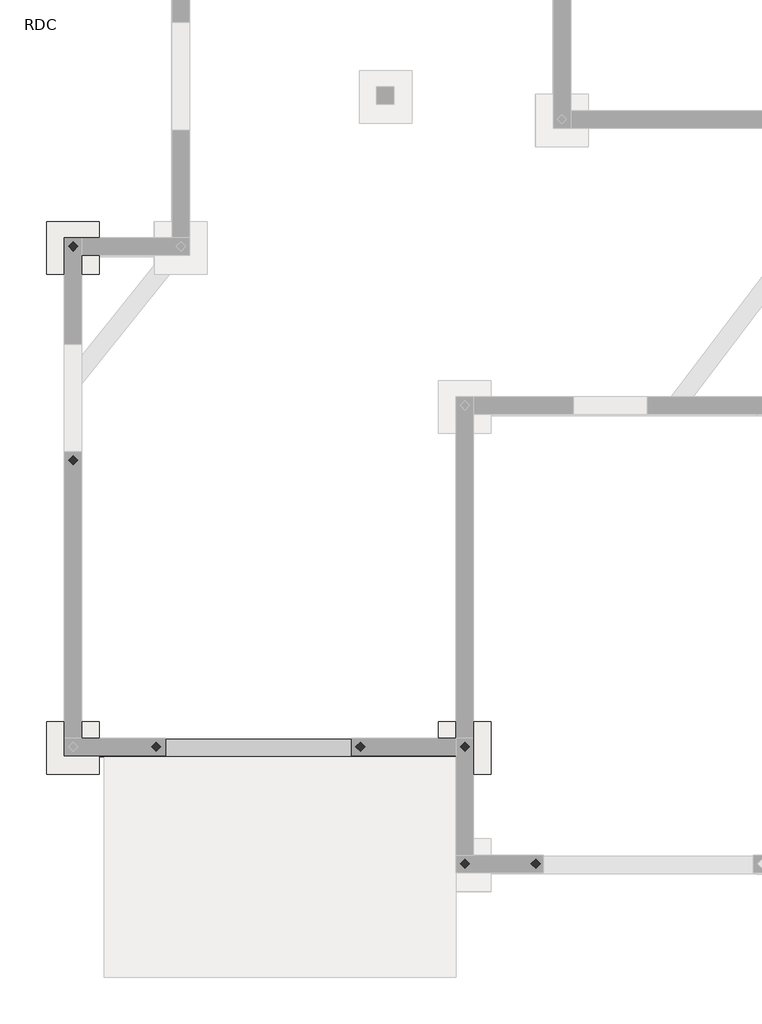
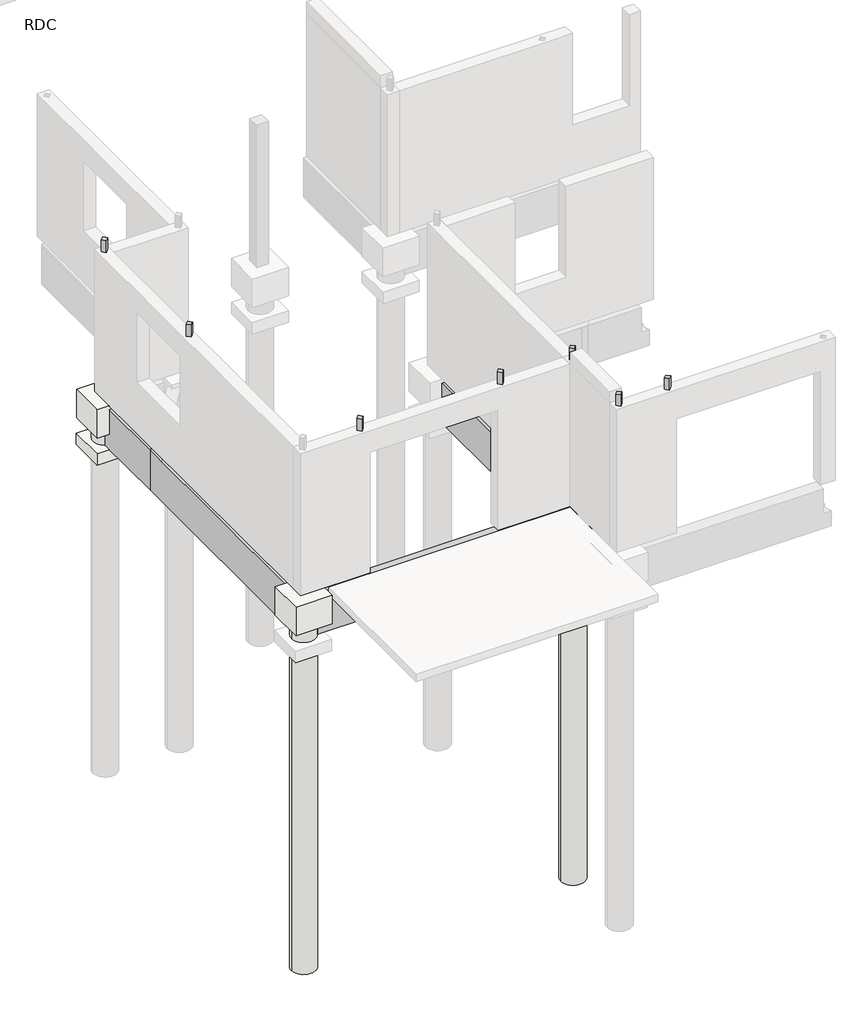
# One storey, part 2 of 5: 7 columns, 7 slabs, 5 beams.
"""IFC4 building model written with IfcOpenShell, lengths in millimetres."""

import ifcopenshell
import ifcopenshell.guid

model = None  # the IFC model being written
_history = None  # IfcOwnerHistory: only IFC2X3 demands one
_inside = {}  # id of a spatial element -> (the spatial element, [elements in it])
_under = {}  # id of a project, library or spatial element -> (it, [spatial elements below it])
_declared = {}  # id of a project -> (the project, [libraries it declares])
_typed = {}  # id of a type object -> (the type object, [elements of that type])
_made_of = {}  # id of a material, layer set ... -> (it, [elements and type objects made of it])


def new_model(schema):
    """Start an empty IFC model of exactly this schema.

    Asked for "IFC4X3", IfcOpenShell would pick the latest addendum, in which some entities
    have other attributes; the version numbers below select the first issue.
    IFC2X3 requires an IfcOwnerHistory on every rooted entity: one is made here for all.
    """
    global model, _history
    if schema == "IFC4X3":
        model = ifcopenshell.file(schema_version=(4, 3, 0, 0))
    else:
        model = ifcopenshell.file(schema=schema)
    _inside.clear()
    _under.clear()
    _declared.clear()
    _typed.clear()
    _made_of.clear()
    _history = None
    if model.schema == "IFC2X3":
        org = make("IfcOrganization", Name="unknown")
        user = make(
            "IfcPersonAndOrganization",
            ThePerson=make("IfcPerson", FamilyName="unknown"),
            TheOrganization=org,
        )
        app = make(
            "IfcApplication",
            ApplicationDeveloper=org,
            Version="unknown",
            ApplicationFullName="unknown",
            ApplicationIdentifier="unknown",
        )
        _history = make(
            "IfcOwnerHistory",
            OwningUser=user,
            OwningApplication=app,
            ChangeAction="ADDED",
            CreationDate=0,
        )
    return model


def make(cls, **values):
    """One entity of the class cls with the attributes given. An attribute that is None is left unset."""
    return model.create_entity(
        cls, **{name: value for name, value in values.items() if value is not None}
    )


def rooted(cls, **values):
    """An entity with a GlobalId (a new one), such as an element, a storey or a relation."""
    return make(cls, GlobalId=ifcopenshell.guid.new(), OwnerHistory=_history, **values)


def si_unit(unit_type, name, prefix=None):
    """IfcSIUnit, for example si_unit("LENGTHUNIT", "METRE", prefix="MILLI")."""
    return make("IfcSIUnit", UnitType=unit_type, Prefix=prefix, Name=name)


def assignment(units):
    """IfcUnitAssignment: the units of a project."""
    return None if units is None else make("IfcUnitAssignment", Units=units)


def point(xyz):
    """IfcCartesianPoint."""
    return None if xyz is None else make("IfcCartesianPoint", Coordinates=xyz)


def direction(xyz):
    """IfcDirection."""
    return None if xyz is None else make("IfcDirection", DirectionRatios=xyz)


def frame(location, z_axis=None, x_axis=None):
    """IfcAxis2Placement3D, a coordinate frame: its origin and axes. An axis left out is left unset."""
    return make(
        "IfcAxis2Placement3D",
        Location=point(location),
        Axis=direction(z_axis),
        RefDirection=direction(x_axis),
    )


def origin():
    """The frame at (0, 0, 0) with its axes left unset."""
    return frame((0.0, 0.0, 0.0))


def place(relative_to, where):
    """IfcLocalPlacement: puts the frame where relative to a parent placement (None: the world)."""
    return make(
        "IfcLocalPlacement", PlacementRelTo=relative_to, RelativePlacement=where
    )


def context(
    kind, dimensions, precision=None, world=None, true_north=None, identifier=None
):
    """IfcGeometricRepresentationContext, for example the 3D "Model" context."""
    return make(
        "IfcGeometricRepresentationContext",
        ContextIdentifier=identifier,
        ContextType=kind,
        CoordinateSpaceDimension=dimensions,
        Precision=precision,
        WorldCoordinateSystem=world,
        TrueNorth=true_north,
    )


def project(units=None, contexts=None):
    """IfcProject with its units and contexts."""
    return rooted(
        "IfcProject",
        Name="project",
        RepresentationContexts=contexts,
        UnitsInContext=assignment(units),
    )


def spatial(cls, under=None, at=None, **own):
    """A site, building, storey or space (cls), placed at a placement, below another one or the project."""
    s = rooted(cls, ObjectPlacement=at, **own)
    if under is not None:
        _under.setdefault(under.id(), (under, []))[1].append(s)
    return s


def polyline(points):
    """IfcPolyline through the points."""
    return make("IfcPolyline", Points=[point(p) for p in points])


def circle_curve(where, radius):
    """IfcCircle in the frame where."""
    return make("IfcCircle", Position=where, Radius=radius)


def outline(outer, holes=None, kind="AREA"):
    """IfcArbitraryClosedProfileDef: a profile drawn as a closed curve; with holes, ...WithVoids."""
    if holes is None:
        return make("IfcArbitraryClosedProfileDef", ProfileType=kind, OuterCurve=outer)
    return make(
        "IfcArbitraryProfileDefWithVoids",
        ProfileType=kind,
        OuterCurve=outer,
        InnerCurves=holes,
    )


def extrude(swept, where, along, depth):
    """IfcExtrudedAreaSolid: the profile swept, set in the frame where, extruded along a direction by depth."""
    return make(
        "IfcExtrudedAreaSolid",
        SweptArea=swept,
        Position=where,
        ExtrudedDirection=direction(along),
        Depth=depth,
    )


def faces_of(points, faces, orient=None, outer=None):
    """IfcFace entities. A face is a list of loops; a loop is a list of indices into points, from 0.

    orient and outer hold one flag for each loop. By default every Orientation is true, the
    first loop of a face is its IfcFaceOuterBound and the others are IfcFaceBound.
    """
    made = []
    for i, loops in enumerate(faces):
        bounds = []
        for j, loop in enumerate(loops):
            is_outer = j == 0 if outer is None else outer[i][j]
            bounds.append(
                make(
                    "IfcFaceOuterBound" if is_outer else "IfcFaceBound",
                    Bound=make("IfcPolyLoop", Polygon=[points[k] for k in loop]),
                    Orientation=True if orient is None else orient[i][j],
                )
            )
        made.append(make("IfcFace", Bounds=bounds))
    return made


def faceted_brep(points, faces, orient=None, outer=None, voids=None):
    """IfcFacetedBrep: a solid bounded by flat faces; with voids (closed shells), ...WithVoids."""
    shared = [point(p) for p in points]
    hull = make("IfcClosedShell", CfsFaces=faces_of(shared, faces, orient, outer))
    if voids is None:
        return make("IfcFacetedBrep", Outer=hull)
    return make(
        "IfcFacetedBrepWithVoids",
        Outer=hull,
        Voids=[
            make(cls, CfsFaces=faces_of(shared, fs, o, b)) for cls, fs, o, b in voids
        ],
    )


def shape(context_of_items, identifier, shape_type, items):
    """IfcShapeRepresentation: the items that make up one representation, for example the "Body"."""
    return make(
        "IfcShapeRepresentation",
        ContextOfItems=context_of_items,
        RepresentationIdentifier=identifier,
        RepresentationType=shape_type,
        Items=items,
    )


def made_of(thing, what):
    """Note that an element or type object is made of a material, layer set ...; save() writes the relation."""
    if what is not None:
        _made_of.setdefault(what.id(), (what, []))[1].append(thing)
    return thing


def element(
    cls,
    number,
    at=None,
    inside=None,
    cuts=None,
    type_object=None,
    material=None,
    context=None,
    identifier="Body",
    shape_type=None,
    held_by="IfcProductDefinitionShape",
    body=None,
    shapes=None,
    **own,
):
    """One element of the class cls, such as IfcWall. Its Tag is "e" and its number.

    at: its placement. inside: the storey or other place that contains it. cuts: it is an
    opening in that element (IfcRelVoidsElement). A single representation is given by context,
    identifier, shape_type and body (its items); several are given by shapes. held_by: the class
    of the entity that holds the representations. save() writes the other relations.
    """
    e = rooted(cls, Tag="e%d" % number, ObjectPlacement=at, **own)
    if body is not None:
        shapes = [shape(context, identifier, shape_type, body)]
    if shapes is not None:
        e.Representation = make(held_by, Representations=shapes)
    if inside is not None:
        _inside.setdefault(inside.id(), (inside, []))[1].append(e)
    if cuts is not None:
        rooted(
            "IfcRelVoidsElement", RelatingBuildingElement=cuts, RelatedOpeningElement=e
        )
    if type_object is not None:
        _typed.setdefault(type_object.id(), (type_object, []))[1].append(e)
    return made_of(e, material)


def aggregate(whole, parts):
    """IfcRelAggregates: a whole, such as a stair, and the parts it consists of."""
    return rooted("IfcRelAggregates", RelatingObject=whole, RelatedObjects=parts)


def save(model, path):
    """Write the relations noted so far, then the file.

    IfcRelAggregates (storeys below a building ...), IfcRelContainedInSpatialStructure (elements
    in a storey), IfcRelDefinesByType, IfcRelAssociatesMaterial and IfcRelDeclares: one each for
    every whole, place, type object, material and project.
    """
    for whole, parts in _under.values():
        aggregate(whole, parts)
    for where, things in _inside.values():
        rooted(
            "IfcRelContainedInSpatialStructure",
            RelatedElements=things,
            RelatingStructure=where,
        )
    for kind, things in _typed.values():
        rooted("IfcRelDefinesByType", RelatedObjects=things, RelatingType=kind)
    for what, things in _made_of.values():
        rooted("IfcRelAssociatesMaterial", RelatedObjects=things, RelatingMaterial=what)
    for by, libraries in _declared.values():
        rooted("IfcRelDeclares", RelatingContext=by, RelatedDefinitions=libraries)
    model.write(path)


def plane_surface(at):
    """IfcPlane: the flat surface through the origin of the frame at, square to its z axis."""
    return make("IfcPlane", Position=at)


def cylinder_surface(at, radius):
    """IfcCylindricalSurface: all points at the distance radius from the z axis of the frame at."""
    return make("IfcCylindricalSurface", Position=at, Radius=radius)


def revolved_surface(curve, axis_point, axis_direction):
    """IfcSurfaceOfRevolution: the curve turned about the line through axis_point along axis_direction."""
    return make(
        "IfcSurfaceOfRevolution",
        SweptCurve=make("IfcArbitraryOpenProfileDef", ProfileType="CURVE", Curve=curve),
        AxisPosition=make("IfcAxis1Placement", Location=point(axis_point), Axis=direction(axis_direction)),
    )


def advanced_brep(points, edges, surfaces, faces):
    """IfcAdvancedBrep: a solid bounded by faces that lie on surfaces and meet in shared edges.

    An edge is (start, end): straight between two places in points (the first is 0);
    or (start, end, curve); or (start, end, curve, False) where it runs against its curve.
    A face is (place in surfaces, loops), or (place, loops, False) where it looks against
    its surface's normal. A loop lists edges by number (the first is 1), with a minus sign
    where the edge is run from its end to its start. The first loop is the outer one.
    """
    corners = [point(p) for p in points]
    vertices = [make("IfcVertexPoint", VertexGeometry=c) for c in corners]
    made = []
    for start, end, *more in edges:
        made.append(
            make(
                "IfcEdgeCurve",
                EdgeStart=vertices[start],
                EdgeEnd=vertices[end],
                EdgeGeometry=more[0] if more else make("IfcPolyline", Points=[corners[start], corners[end]]),
                SameSense=more[1] if len(more) > 1 else True,
            )
        )
    hull = []
    for where, loops, *sense in faces:
        bounds = []
        for j, loop in enumerate(loops):
            ring = [make("IfcOrientedEdge", EdgeElement=made[abs(k) - 1], Orientation=k > 0) for k in loop]
            bounds.append(
                make(
                    "IfcFaceOuterBound" if j == 0 else "IfcFaceBound",
                    Bound=make("IfcEdgeLoop", EdgeList=ring),
                    Orientation=True,
                )
            )
        hull.append(make("IfcAdvancedFace", Bounds=bounds, FaceSurface=surfaces[where], SameSense=sense[0] if sense else True))
    return make("IfcAdvancedBrep", Outer=make("IfcClosedShell", CfsFaces=hull))


model = new_model("IFC4")

# Units and contexts
model_context = context("Model", 3, world=origin())
ifc_project = project(units=[si_unit("LENGTHUNIT", "METRE", prefix="MILLI")], contexts=[model_context])

# Site, building, storey
site = spatial("IfcSite", under=ifc_project)
building = spatial("IfcBuilding", under=site)
storey = spatial("IfcBuildingStorey", under=building, Name="RDC", Elevation=0.0)

# Beams
placement = place(None, origin())
element("IfcBeam", 1, ObjectType="Longrine BA : 20x70ht", at=placement, inside=storey, context=model_context, shape_type="AdvancedBrep", body=[
    advanced_brep(
    [(-6046.4904447, -2179.5386223, -767.0), (-6046.4904447, -2179.5386223, -67.0), (-6046.4904447, -6364.5149728, -67.0), (-6046.4904447, -6364.5149728, -500.0), (-6046.4904447, -6491.309892, -500.0), (-6046.4904447, -6491.309892, -767.0), (-6246.4904447, -6491.309892, -767.0), (-6246.4904447, -2429.4243416, -767.0), (-6246.4904447, -2429.4243416, -67.0), (-6246.4904447, -6491.309892, -500.0), (-6246.4904447, -6364.5149728, -500.0), (-6246.4904447, -6364.5149728, -67.0)],
    [
        (0, 1),
        (1, 2),
        (2, 3),
        (3, 4),
        (4, 5),
        (5, 0),
        (5, 6, circle_curve(frame((-6146.4904447, -6664.5149728, -767.0), z_axis=(0.0, 0.0, 1.0), x_axis=(1.0, 0.0, 0.0)), 200.0)),
        (6, 7),
        (7, 0),
        (8, 7),
        (6, 9),
        (9, 10),
        (10, 11),
        (11, 8),
        (1, 8),
        (11, 2),
        (4, 9, circle_curve(frame((-6146.4904447, -6664.5149728, -500.0), z_axis=(0.0, 0.0, 1.0), x_axis=(1.0, 0.0, 0.0)), 200.0)),
        (3, 10),
    ],
    [
        plane_surface(frame((-6046.4904447, -2539.7018932, -67.0), z_axis=(1.0, 0.0, 0.0), x_axis=(0.0, -1.0, 0.0))),
        plane_surface(frame((-6046.4904447, -2539.7018932, -767.0), z_axis=(0.0, 0.0, -1.0), x_axis=(0.0, -1.0, 0.0))),
        plane_surface(frame((-6246.4904447, -2539.7018932, -767.0), z_axis=(-1.0, 0.0, 0.0), x_axis=(0.0, -1.0, 0.0))),
        plane_surface(frame((-6246.4904447, -2539.7018932, -67.0), z_axis=(0.0, 0.0, 1.0), x_axis=(0.0, -1.0, 0.0))),
        revolved_surface(polyline([(-5946.4904447, -6664.5149728, -500.0), (-5946.4904447, -6664.5149728, -767.0)]), (-6146.4904447, -6664.5149728, -6600.0), (0.0, 0.0, 1.0)),
        plane_surface(frame((-6035.9796689, -2166.4061585, -767.0), z_axis=(-0.7807294524755704, 0.6248692039436703, 0.0), x_axis=(-0.6248692039436703, -0.7807294524755704, 0.0))),
        plane_surface(frame((-6446.4904447, -6364.5149728, -500.0), z_axis=(0.0, 0.0, 1.0), x_axis=(1.0, 0.0, 0.0))),
        plane_surface(frame((-5846.4904447, -6364.5149728, 0.0), z_axis=(0.0, -1.0, 0.0), x_axis=(0.0, 0.0, -1.0))),
    ],
    [
        (0, [[1, 2, 3, 4, 5, 6]]),
        (1, [[7, 8, 9, -6]]),
        (2, [[10, -8, 11, 12, 13, 14]]),
        (3, [[15, -14, 16, -2]]),
        (4, [[-7, -5, 17, -11]]),
        (5, [[-1, -9, -10, -15]]),
        (6, [[18, -12, -17, -4]]),
        (7, [[-18, -3, -16, -13]]),
    ],
),
])
element("IfcBeam", 2, ObjectType="Longrine BA : 20x70ht", at=placement, inside=storey, context=model_context, shape_type="AdvancedBrep", body=[
    advanced_brep(
    [(-1766.4904447, -6491.309892, -767.0), (-1766.4904447, -6491.309892, -500.0), (-1766.4904447, -6364.5149728, -500.0), (-1766.4904447, -6364.5149728, -67.0), (-1766.4904447, -3064.5149728, -67.0), (-1766.4904447, -3064.5149728, -500.0), (-1766.4904447, -2937.7200535, -500.0), (-1766.4904447, -2937.7200535, -767.0), (-1566.4904447, -6491.309892, -767.0), (-1566.4904447, -2937.7200535, -767.0), (-1566.4904447, -6491.309892, -500.0), (-1566.4904447, -2937.7200535, -500.0), (-1566.4904447, -3064.5149728, -500.0), (-1566.4904447, -3064.5149728, -67.0), (-1566.4904447, -6364.5149728, -67.0), (-1566.4904447, -6364.5149728, -500.0)],
    [
        (0, 1),
        (1, 2),
        (2, 3),
        (3, 4),
        (4, 5),
        (5, 6),
        (6, 7),
        (7, 0),
        (8, 0, circle_curve(frame((-1666.4904447, -6664.5149728, -767.0), z_axis=(0.0, 0.0, 1.0), x_axis=(1.0, 0.0, 0.0)), 200.0)),
        (7, 9, circle_curve(frame((-1666.4904447, -2764.5149728, -767.0), z_axis=(0.0, 0.0, 1.0), x_axis=(1.0, 0.0, 0.0)), 200.0)),
        (9, 8),
        (10, 8),
        (9, 11),
        (11, 12),
        (12, 13),
        (13, 14),
        (14, 15),
        (15, 10),
        (3, 14),
        (13, 4),
        (10, 1, circle_curve(frame((-1666.4904447, -6664.5149728, -500.0), z_axis=(0.0, 0.0, 1.0), x_axis=(1.0, 0.0, 0.0)), 200.0)),
        (6, 11, circle_curve(frame((-1666.4904447, -2764.5149728, -500.0), z_axis=(0.0, 0.0, 1.0), x_axis=(1.0, 0.0, 0.0)), 200.0)),
        (15, 2),
        (5, 12),
    ],
    [
        plane_surface(frame((-1766.4904447, -6649.277519, -417.0), z_axis=(-1.0, 0.0, 0.0), x_axis=(0.0, 0.0, -1.0))),
        plane_surface(frame((-1666.4904447, -6649.277519, -767.0), z_axis=(0.0, 0.0, -1.0), x_axis=(1.0, 0.0, 0.0))),
        plane_surface(frame((-1566.4904447, -6649.277519, -417.0), z_axis=(1.0, 0.0, 0.0), x_axis=(0.0, 0.0, 1.0))),
        plane_surface(frame((-1666.4904447, -6649.277519, -67.0), z_axis=(0.0, 0.0, 1.0), x_axis=(-1.0, 0.0, 0.0))),
        revolved_surface(polyline([(-1466.4904447, -6664.5149728, -500.0), (-1466.4904447, -6664.5149728, -767.0)]), (-1666.4904447, -6664.5149728, -6600.0), (0.0, 0.0, 1.0)),
        revolved_surface(polyline([(-1466.4904447, -2764.5149728, -500.0), (-1466.4904447, -2764.5149728, -767.0)]), (-1666.4904447, -2764.5149728, -6600.0), (0.0, 0.0, 1.0)),
        plane_surface(frame((-1966.4904447, -6364.5149728, -500.0), z_axis=(0.0, 0.0, 1.0), x_axis=(1.0, 0.0, 0.0))),
        plane_surface(frame((-1366.4904447, -6364.5149728, 0.0), z_axis=(0.0, -1.0, 0.0), x_axis=(0.0, 0.0, -1.0))),
        plane_surface(frame((-1966.4904447, -2464.5149728, -500.0), z_axis=(0.0, 0.0, 1.0), x_axis=(1.0, 0.0, 0.0))),
        plane_surface(frame((-1966.4904447, -3064.5149728, 0.0), z_axis=(0.0, 1.0, 0.0), x_axis=(0.0, 0.0, -1.0))),
    ],
    [
        (0, [[1, 2, 3, 4, 5, 6, 7, 8]]),
        (1, [[9, -8, 10, 11]]),
        (2, [[12, -11, 13, 14, 15, 16, 17, 18]]),
        (3, [[19, -16, 20, -4]]),
        (4, [[-1, -9, -12, 21]]),
        (5, [[-10, -7, 22, -13]]),
        (6, [[23, -2, -21, -18]]),
        (7, [[-23, -17, -19, -3]]),
        (8, [[24, -14, -22, -6]]),
        (9, [[-24, -5, -20, -15]]),
    ],
),
])
element("IfcBeam", 3, ObjectType="Longrine BA : 20x70ht", at=placement, inside=storey, context=model_context, shape_type="AdvancedBrep", body=[
    advanced_brep(
    [(-1766.4904447, -7828.7724377, -500.0), (-1766.4904447, -7701.9775185, -500.0), (-1766.4904447, -7701.9775185, -67.0), (-1766.4904447, -6964.5149728, -67.0), (-1766.4904447, -6964.5149728, -500.0), (-1766.4904447, -6837.7200535, -500.0), (-1766.4904447, -6837.7200535, -767.0), (-1766.4904447, -7828.7724377, -767.0), (-1566.4904447, -6837.7200535, -767.0), (-1566.4904447, -7828.7724377, -767.0), (-1566.4904447, -7828.7724377, -500.0), (-1566.4904447, -6837.7200535, -500.0), (-1566.4904447, -6964.5149728, -500.0), (-1566.4904447, -6964.5149728, -67.0), (-1566.4904447, -7701.9775185, -67.0), (-1566.4904447, -7701.9775185, -500.0)],
    [
        (0, 1),
        (1, 2),
        (2, 3),
        (3, 4),
        (4, 5),
        (5, 6),
        (6, 7),
        (7, 0),
        (6, 8, circle_curve(frame((-1666.4904447, -6664.5149728, -767.0), z_axis=(0.0, 0.0, 1.0), x_axis=(1.0, 0.0, 0.0)), 200.0)),
        (8, 9),
        (9, 7, circle_curve(frame((-1666.4904447, -8001.9775185, -767.0), z_axis=(0.0, 0.0, 1.0), x_axis=(1.0, 0.0, 0.0)), 200.0)),
        (10, 9),
        (8, 11),
        (11, 12),
        (12, 13),
        (13, 14),
        (14, 15),
        (15, 10),
        (2, 14),
        (13, 3),
        (5, 11, circle_curve(frame((-1666.4904447, -6664.5149728, -500.0), z_axis=(0.0, 0.0, 1.0), x_axis=(1.0, 0.0, 0.0)), 200.0)),
        (10, 0, circle_curve(frame((-1666.4904447, -8001.9775185, -500.0), z_axis=(0.0, 0.0, 1.0), x_axis=(1.0, 0.0, 0.0)), 200.0)),
        (15, 1),
        (4, 12),
    ],
    [
        plane_surface(frame((-1766.4904447, -7989.2775179, -417.0), z_axis=(-1.0, 0.0, 0.0), x_axis=(0.0, 0.0, -1.0))),
        plane_surface(frame((-1666.4904447, -7989.2775179, -767.0), z_axis=(0.0, 0.0, -1.0), x_axis=(1.0, 0.0, 0.0))),
        plane_surface(frame((-1566.4904447, -7989.2775179, -417.0), z_axis=(1.0, 0.0, 0.0), x_axis=(0.0, 0.0, 1.0))),
        plane_surface(frame((-1666.4904447, -7989.2775179, -67.0), z_axis=(0.0, 0.0, 1.0), x_axis=(-1.0, 0.0, 0.0))),
        revolved_surface(polyline([(-1466.4904447, -6664.5149728, -500.0), (-1466.4904447, -6664.5149728, -767.0)]), (-1666.4904447, -6664.5149728, -6600.0), (0.0, 0.0, 1.0)),
        revolved_surface(polyline([(-1466.4904447, -8001.9775185, -500.0), (-1466.4904447, -8001.9775185, -767.0)]), (-1666.4904447, -8001.9775185, -6600.0), (0.0, 0.0, 1.0)),
        plane_surface(frame((-1966.4904447, -7701.9775185, -500.0), z_axis=(0.0, 0.0, 1.0), x_axis=(1.0, 0.0, 0.0))),
        plane_surface(frame((-1366.4904447, -7701.9775185, 0.0), z_axis=(0.0, -1.0, 0.0), x_axis=(0.0, 0.0, -1.0))),
        plane_surface(frame((-1966.4904447, -6364.5149728, -500.0), z_axis=(0.0, 0.0, 1.0), x_axis=(1.0, 0.0, 0.0))),
        plane_surface(frame((-1966.4904447, -6964.5149728, 0.0), z_axis=(0.0, 1.0, 0.0), x_axis=(0.0, 0.0, -1.0))),
    ],
    [
        (0, [[1, 2, 3, 4, 5, 6, 7, 8]]),
        (1, [[9, 10, 11, -7]]),
        (2, [[12, -10, 13, 14, 15, 16, 17, 18]]),
        (3, [[19, -16, 20, -3]]),
        (4, [[-9, -6, 21, -13]]),
        (5, [[-12, 22, -8, -11]]),
        (6, [[23, -1, -22, -18]]),
        (7, [[-23, -17, -19, -2]]),
        (8, [[24, -14, -21, -5]]),
        (9, [[-24, -4, -20, -15]]),
    ],
),
])
element("IfcBeam", 4, ObjectType="Longrine BA : 20x70ht", at=placement, inside=storey, context=model_context, shape_type="AdvancedBrep", body=[
    advanced_brep(
    [(-5974.7753589, -6561.9775197, -767.0), (-5974.7753589, -6561.9775197, -500.0), (-5846.4904447, -6561.9775197, -500.0), (-5846.4904447, -6561.9775197, -67.0), (-1966.4904447, -6561.9775197, -67.0), (-1966.4904447, -6561.9775197, -500.0), (-1838.2055306, -6561.9775197, -500.0), (-1838.2055306, -6561.9775197, -767.0), (-5971.844941, -6761.9775197, -767.0), (-5946.4904447, -6664.5149728, -767.0), (-1866.4904447, -6664.5149728, -767.0), (-1841.1359484, -6761.9775197, -767.0), (-5971.844941, -6761.9775197, -500.0), (-1841.1359484, -6761.9775197, -500.0), (-1966.4904447, -6761.9775197, -500.0), (-1966.4904447, -6761.9775197, -130.0), (-1966.4904447, -6761.9775197, -67.0), (-5789.9771448, -6761.9775197, -67.0), (-5846.4904447, -6761.9775197, -67.0), (-5846.4904447, -6761.9775197, -500.0), (-5946.4904447, -6664.5149728, -500.0), (-1866.4904447, -6664.5149728, -500.0)],
    [
        (0, 1),
        (1, 2),
        (2, 3),
        (3, 4),
        (4, 5),
        (5, 6),
        (6, 7),
        (7, 0),
        (8, 9, circle_curve(frame((-6146.4904447, -6664.5149728, -767.0), z_axis=(0.0, 0.0, 1.0), x_axis=(1.0, 0.0, 0.0)), 200.0)),
        (9, 0, circle_curve(frame((-6146.4904447, -6664.5149728, -767.0), z_axis=(0.0, 0.0, 1.0), x_axis=(1.0, 0.0, 0.0)), 200.0)),
        (7, 10, circle_curve(frame((-1666.4904447, -6664.5149728, -767.0), z_axis=(0.0, 0.0, 1.0), x_axis=(1.0, 0.0, 0.0)), 200.0)),
        (10, 11, circle_curve(frame((-1666.4904447, -6664.5149728, -767.0), z_axis=(0.0, 0.0, 1.0), x_axis=(1.0, 0.0, 0.0)), 200.0)),
        (11, 8),
        (12, 8),
        (11, 13),
        (13, 14),
        (14, 15),
        (15, 16),
        (16, 17),
        (17, 18),
        (18, 19),
        (19, 12),
        (3, 18),
        (16, 4),
        (12, 20, circle_curve(frame((-6146.4904447, -6664.5149728, -500.0), z_axis=(0.0, 0.0, 1.0), x_axis=(1.0, 0.0, 0.0)), 200.0)),
        (20, 9),
        (20, 1, circle_curve(frame((-6146.4904447, -6664.5149728, -500.0), z_axis=(0.0, 0.0, 1.0), x_axis=(1.0, 0.0, 0.0)), 200.0)),
        (10, 21),
        (21, 13, circle_curve(frame((-1666.4904447, -6664.5149728, -500.0), z_axis=(0.0, 0.0, 1.0), x_axis=(1.0, 0.0, 0.0)), 200.0)),
        (6, 21, circle_curve(frame((-1666.4904447, -6664.5149728, -500.0), z_axis=(0.0, 0.0, 1.0), x_axis=(1.0, 0.0, 0.0)), 200.0)),
        (19, 2),
        (5, 14),
    ],
    [
        plane_surface(frame((-6133.7904441, -6561.9775197, -417.0), z_axis=(0.0, 1.0, 0.0), x_axis=(0.0, 0.0, -1.0))),
        plane_surface(frame((-6133.7904441, -6661.9775197, -767.0), z_axis=(0.0, 0.0, -1.0), x_axis=(0.0, -1.0, 0.0))),
        plane_surface(frame((-6133.7904441, -6761.9775197, -417.0), z_axis=(0.0, -1.0, 0.0), x_axis=(0.0, 0.0, 1.0))),
        plane_surface(frame((-6133.7904441, -6661.9775197, -67.0), z_axis=(0.0, 0.0, 1.0), x_axis=(0.0, 1.0, 0.0))),
        revolved_surface(polyline([(-5946.4904447, -6664.5149728, -500.0), (-5946.4904447, -6664.5149728, -767.0)]), (-6146.4904447, -6664.5149728, -6600.0), (0.0, 0.0, 1.0)),
        revolved_surface(polyline([(-1466.4904447, -6664.5149728, -500.0), (-1466.4904447, -6664.5149728, -767.0)]), (-1666.4904447, -6664.5149728, -6600.0), (0.0, 0.0, 1.0)),
        plane_surface(frame((-6446.4904447, -6364.5149728, -500.0), z_axis=(0.0, 0.0, 1.0), x_axis=(1.0, 0.0, 0.0))),
        plane_surface(frame((-5846.4904447, -6964.5149728, 0.0), z_axis=(-1.0, 0.0, 0.0), x_axis=(0.0, 0.0, -1.0))),
        plane_surface(frame((-1966.4904447, -6364.5149728, -500.0), z_axis=(0.0, 0.0, 1.0), x_axis=(1.0, 0.0, 0.0))),
        plane_surface(frame((-1966.4904447, -6364.5149728, 0.0), z_axis=(1.0, 0.0, 0.0), x_axis=(0.0, 0.0, -1.0))),
    ],
    [
        (0, [[1, 2, 3, 4, 5, 6, 7, 8]]),
        (1, [[9, 10, -8, 11, 12, 13]]),
        (2, [[14, -13, 15, 16, 17, 18, 19, 20, 21, 22]]),
        (3, [[23, -20, -19, 24, -4]]),
        (4, [[-14, 25, 26, -9]]),
        (4, [[-1, -10, -26, 27]]),
        (5, [[-12, 28, 29, -15]]),
        (5, [[-11, -7, 30, -28]]),
        (6, [[31, -2, -27, -25, -22]]),
        (7, [[-31, -21, -23, -3]]),
        (8, [[32, -16, -29, -30, -6]]),
        (9, [[-32, -5, -24, -18, -17]]),
    ],
),
])
element("IfcBeam", 5, ObjectType="Longrine BA : 20x70ht", at=placement, inside=storey, context=model_context, shape_type="AdvancedBrep", body=[
    advanced_brep(
    [(-6046.4904447, -1117.578479, -767.0), (-6046.4904447, -1117.578479, -500.0), (-6046.4904447, -1244.3733983, -500.0), (-6046.4904447, -1244.3733983, -67.0), (-6046.4904447, -2179.5386223, -67.0), (-6046.4904447, -2179.5386223, -767.0), (-6246.4904447, -1117.578479, -767.0), (-6246.4904447, -2429.4243416, -767.0), (-6246.4904447, -1117.578479, -500.0), (-6246.4904447, -2429.4243416, -67.0), (-6246.4904447, -1244.3733983, -67.0), (-6246.4904447, -1244.3733983, -500.0)],
    [
        (0, 1),
        (1, 2),
        (2, 3),
        (3, 4),
        (4, 5),
        (5, 0),
        (6, 0, circle_curve(frame((-6146.4904447, -944.3733983, -767.0), z_axis=(0.0, 0.0, 1.0), x_axis=(1.0, 0.0, 0.0)), 200.0)),
        (5, 7),
        (7, 6),
        (8, 6),
        (7, 9),
        (9, 10),
        (10, 11),
        (11, 8),
        (3, 10),
        (9, 4),
        (8, 1, circle_curve(frame((-6146.4904447, -944.3733983, -500.0), z_axis=(0.0, 0.0, 1.0), x_axis=(1.0, 0.0, 0.0)), 200.0)),
        (11, 2),
    ],
    [
        plane_surface(frame((-6046.4904447, -957.0734248, -67.0), z_axis=(1.0, 0.0, 0.0), x_axis=(0.0, -1.0, 0.0))),
        plane_surface(frame((-6046.4904447, -957.0734248, -767.0), z_axis=(0.0, 0.0, -1.0), x_axis=(0.0, -1.0, 0.0))),
        plane_surface(frame((-6246.4904447, -957.0734248, -767.0), z_axis=(-1.0, 0.0, 0.0), x_axis=(0.0, -1.0, 0.0))),
        plane_surface(frame((-6246.4904447, -957.0734248, -67.0), z_axis=(0.0, 0.0, 1.0), x_axis=(0.0, -1.0, 0.0))),
        revolved_surface(polyline([(-5946.4904447, -944.3733983, -500.0), (-5946.4904447, -944.3733983, -767.0)]), (-6146.4904447, -944.3733983, -6600.0), (0.0, 0.0, 1.0)),
        plane_surface(frame((-6446.4904447, -644.3733983, -500.0), z_axis=(0.0, 0.0, 1.0), x_axis=(1.0, 0.0, 0.0))),
        plane_surface(frame((-6446.4904447, -1244.3733983, 0.0), z_axis=(0.0, 1.0, 0.0), x_axis=(0.0, 0.0, -1.0))),
        plane_surface(frame((-6035.9796689, -2166.4061585, -767.0), z_axis=(0.7807294524755704, -0.6248692039436703, 0.0), x_axis=(-0.6248692039436703, -0.7807294524755704, 0.0))),
    ],
    [
        (0, [[1, 2, 3, 4, 5, 6]]),
        (1, [[7, -6, 8, 9]]),
        (2, [[10, -9, 11, 12, 13, 14]]),
        (3, [[15, -12, 16, -4]]),
        (4, [[-1, -7, -10, 17]]),
        (5, [[18, -2, -17, -14]]),
        (6, [[-18, -13, -15, -3]]),
        (7, [[-5, -16, -11, -8]]),
    ],
),
])

# Columns
element("IfcColumn", 6, ObjectType="CV : CV", at=placement, inside=storey, context=model_context, shape_type="Brep", body=[
    faceted_brep([(-1665.4336406, -6595.6690755, 2710.0), (-1718.4666492, -6648.7020841, 2710.0), (-1665.4336406, -6701.7350927, 2710.0), (-1612.400632, -6648.7020841, 2710.0), (-1665.4336406, -6595.6690755, 0.0), (-1612.400632, -6648.7020841, 0.0), (-1665.4336406, -6701.7350927, 0.0), (-1718.4666492, -6648.7020841, 0.0), (-1665.4336406, -6595.6690755, 2500.0), (-1718.4666492, -6648.7020841, 2500.0), (-1665.4336406, -6701.7350927, 2500.0), (-1612.400632, -6648.7020841, 2500.0)], [[[0, 1, 2, 3]], [[4, 5, 6, 7]], [[1, 0, 8, 4, 7, 9]], [[2, 1, 9, 7, 6, 10]], [[3, 2, 10, 6, 5, 11]], [[0, 3, 11, 5, 4, 8]]]),
    faceted_brep([(-1612.400632, -6648.7020841, 2710.0), (-1665.4336406, -6595.6690755, 2710.0), (-1718.4666492, -6648.7020841, 2710.0), (-1665.4336406, -6701.7350927, 2710.0), (-1612.400632, -6648.7020841, 0.0), (-1665.4336406, -6701.7350927, 0.0), (-1718.4666492, -6648.7020841, 0.0), (-1665.4336406, -6595.6690755, 0.0), (-1612.400632, -6648.7020841, 2500.0), (-1665.4336406, -6595.6690755, 2500.0), (-1718.4666492, -6648.7020841, 2500.0), (-1665.4336406, -6701.7350927, 2500.0)], [[[0, 1, 2, 3]], [[4, 5, 6, 7]], [[1, 0, 8, 4, 7, 9]], [[2, 1, 9, 7, 6, 10]], [[3, 2, 10, 6, 5, 11]], [[0, 3, 11, 5, 4, 8]]]),
])
element("IfcColumn", 7, ObjectType="CV : CV", at=placement, inside=storey, context=model_context, shape_type="Brep", body=[
    faceted_brep([(-855.4336191, -7933.1316212, 2710.0), (-908.4666277, -7986.1646298, 2710.0), (-855.4336191, -8039.1976384, 2710.0), (-802.4006105, -7986.1646298, 2710.0), (-855.4336191, -7933.1316212, 0.0), (-802.4006105, -7986.1646298, 0.0), (-855.4336191, -8039.1976384, 0.0), (-908.4666277, -7986.1646298, 0.0), (-855.4336191, -7933.1316212, 2510.0), (-908.4666277, -7986.1646298, 2510.0), (-855.4336191, -8039.1976384, 2510.0), (-802.4006105, -7986.1646298, 2510.0)], [[[0, 1, 2, 3]], [[4, 5, 6, 7]], [[1, 0, 8, 4, 7, 9]], [[2, 1, 9, 7, 6, 10]], [[3, 2, 10, 6, 5, 11]], [[0, 3, 11, 5, 4, 8]]]),
    faceted_brep([(-802.4006105, -7986.1646298, 2710.0), (-855.4336191, -7933.1316212, 2710.0), (-908.4666277, -7986.1646298, 2710.0), (-855.4336191, -8039.1976384, 2710.0), (-802.4006105, -7986.1646298, 0.0), (-855.4336191, -8039.1976384, 0.0), (-908.4666277, -7986.1646298, 0.0), (-855.4336191, -7933.1316212, 0.0), (-802.4006105, -7986.1646298, 2510.0), (-855.4336191, -7933.1316212, 2510.0), (-908.4666277, -7986.1646298, 2510.0), (-855.4336191, -8039.1976384, 2510.0)], [[[0, 1, 2, 3]], [[4, 5, 6, 7]], [[1, 0, 8, 4, 7, 9]], [[2, 1, 9, 7, 6, 10]], [[3, 2, 10, 6, 5, 11]], [[0, 3, 11, 5, 4, 8]]]),
])
element("IfcColumn", 8, ObjectType="CV : CV", at=placement, inside=storey, context=model_context, shape_type="Brep", body=[
    faceted_brep([(-1665.4336406, -7933.1316212, 2710.0), (-1718.4666492, -7986.1646298, 2710.0), (-1665.4336406, -8039.1976384, 2710.0), (-1612.400632, -7986.1646298, 2710.0), (-1665.4336406, -7933.1316212, 0.0), (-1612.400632, -7986.1646298, 0.0), (-1665.4336406, -8039.1976384, 0.0), (-1718.4666492, -7986.1646298, 0.0), (-1665.4336406, -7933.1316212, 2510.0), (-1718.4666492, -7986.1646298, 2510.0), (-1665.4336406, -8039.1976384, 2510.0), (-1612.400632, -7986.1646298, 2510.0)], [[[0, 1, 2, 3]], [[4, 5, 6, 7]], [[1, 0, 8, 4, 7, 9]], [[2, 1, 9, 7, 6, 10]], [[3, 2, 10, 6, 5, 11]], [[0, 3, 11, 5, 4, 8]]]),
    faceted_brep([(-1612.400632, -7986.1646298, 2710.0), (-1665.4336406, -7933.1316212, 2710.0), (-1718.4666492, -7986.1646298, 2710.0), (-1665.4336406, -8039.1976384, 2710.0), (-1612.400632, -7986.1646298, 0.0), (-1665.4336406, -8039.1976384, 0.0), (-1718.4666492, -7986.1646298, 0.0), (-1665.4336406, -7933.1316212, 0.0), (-1612.400632, -7986.1646298, 2510.0), (-1665.4336406, -7933.1316212, 2510.0), (-1718.4666492, -7986.1646298, 2510.0), (-1665.4336406, -8039.1976384, 2510.0)], [[[0, 1, 2, 3]], [[4, 5, 6, 7]], [[1, 0, 8, 4, 7, 9]], [[2, 1, 9, 7, 6, 10]], [[3, 2, 10, 6, 5, 11]], [[0, 3, 11, 5, 4, 8]]]),
])
element("IfcColumn", 9, ObjectType="CV : CV", at=placement, inside=storey, context=model_context, shape_type="Brep", body=[
    faceted_brep([(-2861.4904447, -6595.6690755, 2710.0), (-2914.5234533, -6648.7020841, 2710.0), (-2861.4904447, -6701.7350927, 2710.0), (-2808.4574361, -6648.7020841, 2710.0), (-2861.4904447, -6595.6690755, 0.0), (-2808.4574361, -6648.7020841, 0.0), (-2861.4904447, -6701.7350927, 0.0), (-2914.5234533, -6648.7020841, 0.0), (-2861.4904447, -6595.6690755, 2500.0), (-2914.5234533, -6648.7020841, 2500.0), (-2861.4904447, -6701.7350927, 2500.0), (-2808.4574361, -6648.7020841, 2500.0)], [[[0, 1, 2, 3]], [[4, 5, 6, 7]], [[1, 0, 8, 4, 7, 9]], [[2, 1, 9, 7, 6, 10]], [[3, 2, 10, 6, 5, 11]], [[0, 3, 11, 5, 4, 8]]]),
    faceted_brep([(-2808.4574361, -6648.7020841, 2710.0), (-2861.4904447, -6595.6690755, 2710.0), (-2914.5234533, -6648.7020841, 2710.0), (-2861.4904447, -6701.7350927, 2710.0), (-2808.4574361, -6648.7020841, 0.0), (-2861.4904447, -6701.7350927, 0.0), (-2914.5234533, -6648.7020841, 0.0), (-2861.4904447, -6595.6690755, 0.0), (-2808.4574361, -6648.7020841, 2500.0), (-2861.4904447, -6595.6690755, 2500.0), (-2914.5234533, -6648.7020841, 2500.0), (-2861.4904447, -6701.7350927, 2500.0)], [[[0, 1, 2, 3]], [[4, 5, 6, 7]], [[1, 0, 8, 4, 7, 9]], [[2, 1, 9, 7, 6, 10]], [[3, 2, 10, 6, 5, 11]], [[0, 3, 11, 5, 4, 8]]]),
])
element("IfcColumn", 10, ObjectType="CV : CV", at=placement, inside=storey, context=model_context, shape_type="Brep", body=[
    faceted_brep([(-5197.6214092, -6595.6690755, 2710.0), (-5250.6544178, -6648.7020841, 2710.0), (-5197.6214092, -6701.7350927, 2710.0), (-5144.5884006, -6648.7020841, 2710.0), (-5197.6214092, -6595.6690755, 0.0), (-5144.5884006, -6648.7020841, 0.0), (-5197.6214092, -6701.7350927, 0.0), (-5250.6544178, -6648.7020841, 0.0), (-5197.6214092, -6595.6690755, 2500.0), (-5250.6544178, -6648.7020841, 2500.0), (-5197.6214092, -6701.7350927, 2500.0), (-5144.5884006, -6648.7020841, 2500.0)], [[[0, 1, 2, 3]], [[4, 5, 6, 7]], [[1, 0, 8, 4, 7, 9]], [[2, 1, 9, 7, 6, 10]], [[3, 2, 10, 6, 5, 11]], [[0, 3, 11, 5, 4, 8]]]),
    faceted_brep([(-5144.5884006, -6648.7020841, 2710.0), (-5197.6214092, -6595.6690755, 2710.0), (-5250.6544178, -6648.7020841, 2710.0), (-5197.6214092, -6701.7350927, 2710.0), (-5144.5884006, -6648.7020841, 0.0), (-5197.6214092, -6701.7350927, 0.0), (-5250.6544178, -6648.7020841, 0.0), (-5197.6214092, -6595.6690755, 0.0), (-5144.5884006, -6648.7020841, 2500.0), (-5197.6214092, -6595.6690755, 2500.0), (-5250.6544178, -6648.7020841, 2500.0), (-5197.6214092, -6701.7350927, 2500.0)], [[[0, 1, 2, 3]], [[4, 5, 6, 7]], [[1, 0, 8, 4, 7, 9]], [[2, 1, 9, 7, 6, 10]], [[3, 2, 10, 6, 5, 11]], [[0, 3, 11, 5, 4, 8]]]),
])
element("IfcColumn", 11, ObjectType="CV : CV", at=placement, inside=storey, context=model_context, shape_type="Brep", body=[
    faceted_brep([(-6146.4904447, -3320.5275198, 2710.0), (-6199.5234533, -3373.5605284, 2710.0), (-6146.4904447, -3426.593537, 2710.0), (-6093.4574361, -3373.5605284, 2710.0), (-6146.4904447, -3320.5275198, 0.0), (-6093.4574361, -3373.5605284, 0.0), (-6146.4904447, -3426.593537, 0.0), (-6199.5234533, -3373.5605284, 0.0), (-6146.4904447, -3320.5275198, 2500.0), (-6199.5234533, -3373.5605284, 2500.0), (-6146.4904447, -3426.593537, 2500.0), (-6093.4574361, -3373.5605284, 2500.0)], [[[0, 1, 2, 3]], [[4, 5, 6, 7]], [[1, 0, 8, 4, 7, 9]], [[2, 1, 9, 7, 6, 10]], [[3, 2, 10, 6, 5, 11]], [[0, 3, 11, 5, 4, 8]]]),
    faceted_brep([(-6093.4574361, -3373.5605284, 2710.0), (-6146.4904447, -3320.5275198, 2710.0), (-6199.5234533, -3373.5605284, 2710.0), (-6146.4904447, -3426.593537, 2710.0), (-6093.4574361, -3373.5605284, 0.0), (-6146.4904447, -3426.593537, 0.0), (-6199.5234533, -3373.5605284, 0.0), (-6146.4904447, -3320.5275198, 0.0), (-6093.4574361, -3373.5605284, 2500.0), (-6146.4904447, -3320.5275198, 2500.0), (-6199.5234533, -3373.5605284, 2500.0), (-6146.4904447, -3426.593537, 2500.0)], [[[0, 1, 2, 3]], [[4, 5, 6, 7]], [[1, 0, 8, 4, 7, 9]], [[2, 1, 9, 7, 6, 10]], [[3, 2, 10, 6, 5, 11]], [[0, 3, 11, 5, 4, 8]]]),
])
element("IfcColumn", 12, ObjectType="CV : CV", at=placement, inside=storey, context=model_context, shape_type="Brep", body=[
    faceted_brep([(-6146.4904447, -875.527527, 2710.0), (-6199.5234533, -928.5605356, 2710.0), (-6146.4904447, -981.5935442, 2710.0), (-6093.4574361, -928.5605356, 2710.0), (-6146.4904447, -875.527527, 0.0), (-6093.4574361, -928.5605356, 0.0), (-6146.4904447, -981.5935442, 0.0), (-6199.5234533, -928.5605356, 0.0), (-6146.4904447, -875.527527, 2500.0), (-6199.5234533, -928.5605356, 2500.0), (-6146.4904447, -981.5935442, 2500.0), (-6093.4574361, -928.5605356, 2500.0)], [[[0, 1, 2, 3]], [[4, 5, 6, 7]], [[1, 0, 8, 4, 7, 9]], [[2, 1, 9, 7, 6, 10]], [[3, 2, 10, 6, 5, 11]], [[0, 3, 11, 5, 4, 8]]]),
    faceted_brep([(-6093.4574361, -928.5605356, 2710.0), (-6146.4904447, -875.527527, 2710.0), (-6199.5234533, -928.5605356, 2710.0), (-6146.4904447, -981.5935442, 2710.0), (-6093.4574361, -928.5605356, 0.0), (-6146.4904447, -981.5935442, 0.0), (-6199.5234533, -928.5605356, 0.0), (-6146.4904447, -875.527527, 0.0), (-6093.4574361, -928.5605356, 2500.0), (-6146.4904447, -875.527527, 2500.0), (-6199.5234533, -928.5605356, 2500.0), (-6146.4904447, -981.5935442, 2500.0)], [[[0, 1, 2, 3]], [[4, 5, 6, 7]], [[1, 0, 8, 4, 7, 9]], [[2, 1, 9, 7, 6, 10]], [[3, 2, 10, 6, 5, 11]], [[0, 3, 11, 5, 4, 8]]]),
])

# Slabs
element("IfcSlab", 13, ObjectType="Pieu-Conduite en acier : Diamètre de 400 mm", at=placement, inside=storey, context=model_context, shape_type="AdvancedBrep", body=[
    advanced_brep(
    [(-6346.4904447, -6664.5149728, -6600.0), (-5946.4904447, -6664.5149728, -6600.0), (-6346.4904447, -6664.5149728, -970.0), (-5946.4904447, -6664.5149728, -970.0)],
    [
        (0, 1, circle_curve(frame((-6146.4904447, -6664.5149728, -6600.0), z_axis=(0.0, 0.0, -1.0), x_axis=(1.0, 0.0, 0.0)), 200.0)),
        (1, 0, circle_curve(frame((-6146.4904447, -6664.5149728, -6600.0), z_axis=(0.0, 0.0, -1.0), x_axis=(1.0, 0.0, 0.0)), 200.0)),
        (2, 3, circle_curve(frame((-6146.4904447, -6664.5149728, -970.0), z_axis=(0.0, 0.0, 1.0), x_axis=(1.0, 0.0, 0.0)), 200.0)),
        (3, 2, circle_curve(frame((-6146.4904447, -6664.5149728, -970.0), z_axis=(0.0, 0.0, 1.0), x_axis=(1.0, 0.0, 0.0)), 200.0)),
        (1, 3),
        (2, 0),
    ],
    [
        plane_surface(frame((-5946.4904447, -6664.5149728, -6600.0), z_axis=(0.0, 0.0, -1.0), x_axis=(0.0, -1.0, 0.0))),
        plane_surface(frame((-6451.0339778, -6364.5149728, -970.0), z_axis=(0.0, 0.0, 1.0), x_axis=(1.0, 0.0, 0.0))),
        cylinder_surface(frame((-6146.4904447, -6664.5149728, -6600.0), z_axis=(0.0, 0.0, 1.0), x_axis=(1.0, 0.0, 0.0)), 200.0),
    ],
    [
        (0, [[1, 2]]),
        (1, [[3, 4]]),
        (2, [[-2, 5, -3, 6]]),
        (2, [[-1, -6, -4, -5]]),
    ],
),
    advanced_brep(
    [(-6346.4904447, -6664.5149728, -770.0), (-5946.4904447, -6664.5149728, -770.0), (-5946.4904447, -6664.5149728, -500.0), (-5971.844941, -6761.9775197, -500.0), (-6346.4904447, -6664.5149728, -500.0), (-6246.4904447, -6491.309892, -500.0), (-6046.4904447, -6491.309892, -500.0), (-5974.7836363, -6561.9636591, -500.0)],
    [
        (0, 1, circle_curve(frame((-6146.4904447, -6664.5149728, -770.0), z_axis=(0.0, 0.0, 1.0), x_axis=(1.0, 0.0, 0.0)), 200.0)),
        (1, 2),
        (2, 3, circle_curve(frame((-6146.4904447, -6664.5149728, -500.0), z_axis=(0.0, 0.0, -1.0), x_axis=(1.0, 0.0, 0.0)), 200.0)),
        (3, 4, circle_curve(frame((-6146.4904447, -6664.5149728, -500.0), z_axis=(0.0, 0.0, -1.0), x_axis=(1.0, 0.0, 0.0)), 200.0)),
        (4, 0),
        (1, 0, circle_curve(frame((-6146.4904447, -6664.5149728, -770.0), z_axis=(0.0, 0.0, 1.0), x_axis=(1.0, 0.0, 0.0)), 200.0)),
        (4, 5, circle_curve(frame((-6146.4904447, -6664.5149728, -500.0), z_axis=(0.0, 0.0, -1.0), x_axis=(1.0, 0.0, 0.0)), 200.0)),
        (5, 6, circle_curve(frame((-6146.4904447, -6664.5149728, -500.0), z_axis=(0.0, 0.0, -1.0), x_axis=(1.0, 0.0, 0.0)), 200.0)),
        (6, 7, circle_curve(frame((-6146.4904447, -6664.5149728, -500.0), z_axis=(0.0, 0.0, -1.0), x_axis=(1.0, 0.0, 0.0)), 200.0)),
        (7, 2, circle_curve(frame((-6146.4904447, -6664.5149728, -500.0), z_axis=(0.0, 0.0, -1.0), x_axis=(1.0, 0.0, 0.0)), 200.0)),
    ],
    [
        cylinder_surface(frame((-6146.4904447, -6664.5149728, -6600.0), z_axis=(0.0, 0.0, 1.0), x_axis=(1.0, 0.0, 0.0)), 200.0),
        plane_surface(frame((-6451.0339778, -6364.5149728, -770.0), z_axis=(0.0, 0.0, -1.0), x_axis=(-1.0, 0.0, 0.0))),
        plane_surface(frame((-6446.4904447, -6364.5149728, -500.0), z_axis=(0.0, 0.0, 1.0), x_axis=(1.0, 0.0, 0.0))),
    ],
    [
        (0, [[1, 2, 3, 4, 5]]),
        (0, [[6, -5, 7, 8, 9, 10, -2]]),
        (1, [[-1, -6]]),
        (2, [[-4, -3, -10, -9, -8, -7]]),
    ],
),
])
element("IfcSlab", 14, ObjectType="Pieu-Conduite en acier : Diamètre de 400 mm", at=placement, inside=storey, context=model_context, shape_type="AdvancedBrep", body=[
    advanced_brep(
    [(-1866.4904447, -6664.5149728, -6600.0), (-1466.4904447, -6664.5149728, -6600.0), (-1866.4904447, -6664.5149728, -970.0), (-1466.4904447, -6664.5149728, -970.0)],
    [
        (0, 1, circle_curve(frame((-1666.4904447, -6664.5149728, -6600.0), z_axis=(0.0, 0.0, -1.0), x_axis=(1.0, 0.0, 0.0)), 200.0)),
        (1, 0, circle_curve(frame((-1666.4904447, -6664.5149728, -6600.0), z_axis=(0.0, 0.0, -1.0), x_axis=(1.0, 0.0, 0.0)), 200.0)),
        (2, 3, circle_curve(frame((-1666.4904447, -6664.5149728, -970.0), z_axis=(0.0, 0.0, 1.0), x_axis=(1.0, 0.0, 0.0)), 200.0)),
        (3, 2, circle_curve(frame((-1666.4904447, -6664.5149728, -970.0), z_axis=(0.0, 0.0, 1.0), x_axis=(1.0, 0.0, 0.0)), 200.0)),
        (1, 3),
        (2, 0),
    ],
    [
        plane_surface(frame((-1466.4904447, -6664.5149728, -6600.0), z_axis=(0.0, 0.0, -1.0), x_axis=(0.0, -1.0, 0.0))),
        plane_surface(frame((-1969.9771566, -6364.5149728, -970.0), z_axis=(0.0, 0.0, 1.0), x_axis=(1.0, 0.0, 0.0))),
        cylinder_surface(frame((-1666.4904447, -6664.5149728, -6600.0), z_axis=(0.0, 0.0, 1.0), x_axis=(1.0, 0.0, 0.0)), 200.0),
    ],
    [
        (0, [[1, 2]]),
        (1, [[3, 4]]),
        (2, [[-2, 5, -3, 6]]),
        (2, [[-1, -6, -4, -5]]),
    ],
),
    advanced_brep(
    [(-1866.4904447, -6664.5149728, -770.0), (-1466.4904447, -6664.5149728, -770.0), (-1466.4904447, -6664.5149728, -500.0), (-1566.4904447, -6837.7200535, -500.0), (-1766.4904447, -6837.7200535, -500.0), (-1841.127419, -6761.9928022, -500.0), (-1866.4904447, -6664.5149728, -500.0), (-1838.1972532, -6561.9636591, -500.0), (-1766.4904447, -6491.309892, -500.0), (-1566.4904447, -6491.309892, -500.0)],
    [
        (0, 1, circle_curve(frame((-1666.4904447, -6664.5149728, -770.0), z_axis=(0.0, 0.0, 1.0), x_axis=(1.0, 0.0, 0.0)), 200.0)),
        (1, 2),
        (2, 3, circle_curve(frame((-1666.4904447, -6664.5149728, -500.0), z_axis=(0.0, 0.0, -1.0), x_axis=(1.0, 0.0, 0.0)), 200.0)),
        (3, 4, circle_curve(frame((-1666.4904447, -6664.5149728, -500.0), z_axis=(0.0, 0.0, -1.0), x_axis=(1.0, 0.0, 0.0)), 200.0)),
        (4, 5, circle_curve(frame((-1666.4904447, -6664.5149728, -500.0), z_axis=(0.0, 0.0, -1.0), x_axis=(1.0, 0.0, 0.0)), 200.0)),
        (5, 6, circle_curve(frame((-1666.4904447, -6664.5149728, -500.0), z_axis=(0.0, 0.0, -1.0), x_axis=(1.0, 0.0, 0.0)), 200.0)),
        (6, 0),
        (1, 0, circle_curve(frame((-1666.4904447, -6664.5149728, -770.0), z_axis=(0.0, 0.0, 1.0), x_axis=(1.0, 0.0, 0.0)), 200.0)),
        (6, 7, circle_curve(frame((-1666.4904447, -6664.5149728, -500.0), z_axis=(0.0, 0.0, -1.0), x_axis=(1.0, 0.0, 0.0)), 200.0)),
        (7, 8, circle_curve(frame((-1666.4904447, -6664.5149728, -500.0), z_axis=(0.0, 0.0, -1.0), x_axis=(1.0, 0.0, 0.0)), 200.0)),
        (8, 9, circle_curve(frame((-1666.4904447, -6664.5149728, -500.0), z_axis=(0.0, 0.0, -1.0), x_axis=(1.0, 0.0, 0.0)), 200.0)),
        (9, 2, circle_curve(frame((-1666.4904447, -6664.5149728, -500.0), z_axis=(0.0, 0.0, -1.0), x_axis=(1.0, 0.0, 0.0)), 200.0)),
    ],
    [
        cylinder_surface(frame((-1666.4904447, -6664.5149728, -6600.0), z_axis=(0.0, 0.0, 1.0), x_axis=(1.0, 0.0, 0.0)), 200.0),
        plane_surface(frame((-1969.9771566, -6364.5149728, -770.0), z_axis=(0.0, 0.0, -1.0), x_axis=(-1.0, 0.0, 0.0))),
        plane_surface(frame((-1966.4904447, -6364.5149728, -500.0), z_axis=(0.0, 0.0, 1.0), x_axis=(1.0, 0.0, 0.0))),
    ],
    [
        (0, [[1, 2, 3, 4, 5, 6, 7]]),
        (0, [[8, -7, 9, 10, 11, 12, -2]]),
        (1, [[-1, -8]]),
        (2, [[-6, -5, -4, -3, -12, -11, -10, -9]]),
    ],
),
])
element("IfcSlab", 15, ObjectType="Tête de pieux-1 poteau : 60x60x50", at=placement, inside=storey, context=model_context, shape_type="Brep", body=[
    faceted_brep([(-5846.4904447, -6364.5149728, 0.0), (-6446.4904447, -6364.5149728, 0.0), (-6446.4904447, -6964.5149728, 0.0), (-5846.4904447, -6964.5149728, 0.0), (-5846.4904447, -6364.5149728, -500.0), (-5846.4904447, -6561.9775197, -500.0), (-5846.4904447, -6761.9775197, -500.0), (-5846.4904447, -6964.5149728, -500.0), (-6446.4904447, -6964.5149728, -500.0), (-6446.4904447, -6364.5149728, -500.0), (-6246.4904447, -6364.5149728, -500.0), (-6046.4904447, -6364.5149728, -500.0)], [[[0, 1, 2, 3]], [[4, 5, 6, 7, 8, 9, 10, 11]], [[1, 0, 4, 11, 10, 9]], [[2, 1, 9, 8]], [[3, 2, 8, 7]], [[0, 3, 7, 6, 5, 4]]]),
])
element("IfcSlab", 16, ObjectType="Tête de pieux-1 poteau : 60x60x50", at=placement, inside=storey, context=model_context, shape_type="Brep", body=[
    faceted_brep([(-1366.4904447, -6364.5149728, 0.0), (-1966.4904447, -6364.5149728, 0.0), (-1966.4904447, -6964.5149728, 0.0), (-1366.4904447, -6964.5149728, 0.0), (-1366.4904447, -6364.5149728, -500.0), (-1366.4904447, -6964.5149728, -500.0), (-1566.4904447, -6964.5149728, -500.0), (-1766.4904447, -6964.5149728, -500.0), (-1966.4904447, -6964.5149728, -500.0), (-1966.4904447, -6761.9775197, -500.0), (-1966.4904447, -6561.9775197, -500.0), (-1966.4904447, -6364.5149728, -500.0), (-1766.4904447, -6364.5149728, -500.0), (-1566.4904447, -6364.5149728, -500.0)], [[[0, 1, 2, 3]], [[4, 5, 6, 7, 8, 9, 10, 11, 12, 13]], [[1, 0, 4, 13, 12, 11]], [[2, 1, 11, 10, 9, 8]], [[3, 2, 8, 7, 6, 5]], [[0, 3, 5, 4]]]),
])
element("IfcSlab", 17, ObjectType="Tête de pieux-1 poteau : 60x60x50", at=placement, inside=storey, context=model_context, shape_type="Brep", body=[
    faceted_brep([(-5846.4904447, -644.3733983, 0.0), (-6446.4904447, -644.3733983, 0.0), (-6446.4904447, -1244.3733983, 0.0), (-5846.4904447, -1244.3733983, 0.0), (-5846.4904447, -644.3733983, -500.0), (-5846.4904447, -844.3734242, -500.0), (-5846.4904447, -1044.3734242, -500.0), (-5846.4904447, -1244.3733983, -500.0), (-6046.4904447, -1244.3733983, -500.0), (-6246.4904447, -1244.3733983, -500.0), (-6446.4904447, -1244.3733983, -500.0), (-6446.4904447, -644.3733983, -500.0)], [[[0, 1, 2, 3]], [[4, 5, 6, 7, 8, 9, 10, 11]], [[1, 0, 4, 11]], [[2, 1, 11, 10]], [[3, 2, 10, 9, 8, 7]], [[0, 3, 7, 6, 5, 4]]]),
])
element("IfcSlab", 18, ObjectType="M_Base-Rectangulaire : 60x60x20", at=placement, inside=storey, context=model_context, shape_type="SweptSolid", body=[
    extrude(outline(polyline([(-1369.9771566, -6364.5149728), (-1369.9771566, -6964.5149728), (-1969.9771566, -6964.5149728), (-1969.9771566, -6364.5149728), (-1369.9771566, -6364.5149728)])), frame((0.0, 0.0, -970.0), z_axis=(0.0, 0.0, 1.0), x_axis=(1.0, 0.0, 0.0)), (0.0, 0.0, 1.0), 200.0),
    extrude(outline(polyline([(-1369.9771566, -6364.5149728), (-1369.9771566, -6964.5149728), (-1969.9771566, -6964.5149728), (-1969.9771566, -6364.5149728), (-1369.9771566, -6364.5149728)])), frame((0.0, 0.0, -970.0), z_axis=(0.0, 0.0, 1.0), x_axis=(1.0, 0.0, 0.0)), (0.0, 0.0, 1.0), 200.0),
])
element("IfcSlab", 19, ObjectType="M_Base-Rectangulaire : 60x60x20", at=placement, inside=storey, context=model_context, shape_type="SweptSolid", body=[
    extrude(outline(polyline([(-5851.0339778, -644.3734242), (-5851.0339778, -1244.3734242), (-6451.0339778, -1244.3734242), (-6451.0339778, -644.3734242), (-5851.0339778, -644.3734242)])), frame((0.0, 0.0, -970.0), z_axis=(0.0, 0.0, 1.0), x_axis=(1.0, 0.0, 0.0)), (0.0, 0.0, 1.0), 200.0),
    extrude(outline(polyline([(-5851.0339778, -644.3734242), (-5851.0339778, -1244.3734242), (-6451.0339778, -1244.3734242), (-6451.0339778, -644.3734242), (-5851.0339778, -644.3734242)])), frame((0.0, 0.0, -970.0), z_axis=(0.0, 0.0, 1.0), x_axis=(1.0, 0.0, 0.0)), (0.0, 0.0, 1.0), 200.0),
])

save(model, "model.ifc")

# Revit data of these elements
# Type "Longrine BA : 20x70ht"
#   Length [instance default] = 1.524 m
#   b = 0.200 m
#   h = 0.700 m
#   Structural Material = Maçonnerie - Béton
#   Assembly Code = ""
# Type "CV : CV"
#   Structural Material [instance default] = Béton coulé sur place
#   Default Elevation = 0
# Type "Pieu-Conduite en acier : Diamètre de 400 mm"
#   Assembly Code = "A1020130"
#   Rayon = 0.200 m
#   Enrobage minimum = 0.150 m
#   Diameter = 0.400 m
#   Depth = 6.000 m
#   Structural Material [instance default] = Métal - Acier - 345 MPa
# Type "Tête de pieux-1 poteau : 60x60x50"
#   Assembly Code = "A1010130"
#   Width = 0.600 m
#   Length = 0.600 m
#   Foundation Thickness = 0.500 m
#   Coupure = 0.050 m
#   Structural Material [instance default] = Béton - Béton coulé sur place
#   Type de pieu = Pieu-Conduite en acier : Diamètre de 400 mm
# Type "M_Base-Rectangulaire : 60x60x20"
#   Length = 0.600 m
#   Width = 0.600 m
#   Foundation Thickness = 0.200 m
#   Structural Material [instance default] = Béton - Béton coulé sur place
#   Assembly Code = ""
# Elements 1, 2, 3, 4, 5 (IfcBeam, "Longrine BA : 20x70ht")
#   Phase Created = Nouvelle construction
#   Materials on its faces: "Maçonnerie - Béton"
# Elements 6, 7, 8, 9, 10, 11, 12 (IfcColumn, "CV : CV")
#   Structural Material = Béton coulé sur place
#   Phase Created = Nouvelle construction
#   Materials on its faces: "Béton coulé sur place"
# Elements 13, 14 (IfcSlab, "Pieu-Conduite en acier : Diamètre de 400 mm")
#   Structural Material = none
#   Phase Created = Nouvelle construction
# Elements 15, 16, 17 (IfcSlab, "Tête de pieux-1 poteau : 60x60x50")
#   Structural Material = Béton - Béton coulé sur place
#   Phase Created = Nouvelle construction
#   Materials on its faces: "Béton - Béton coulé sur place"
# Elements 18, 19 (IfcSlab, "M_Base-Rectangulaire : 60x60x20")
#   Structural Material = Béton - Béton coulé sur place
#   Phase Created = Nouvelle construction
#   Materials on its faces: "Béton - Béton coulé sur place"
# Materials
#   "Maçonnerie - Béton": class "Béton", colour RGB 153 162 160, transparency 0, Cost = 0
#   "Béton coulé sur place": class "Béton", colour RGB 0 0 0, transparency 0, Description = "Matériau physique.", Cost = 0
#   "Métal - Acier - 345 MPa": class "Métal", colour RGB 247 247 247, transparency 0, Cost = 0
#   "Béton - Béton coulé sur place": class "Béton", colour RGB 192 192 192, transparency 0, Cost = 0
